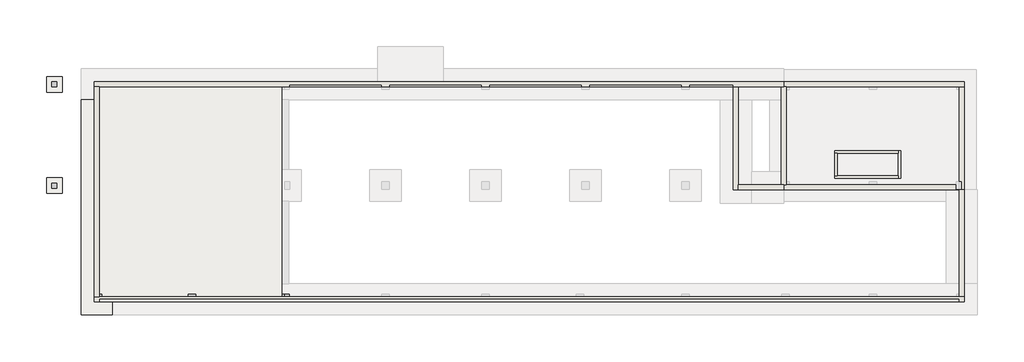
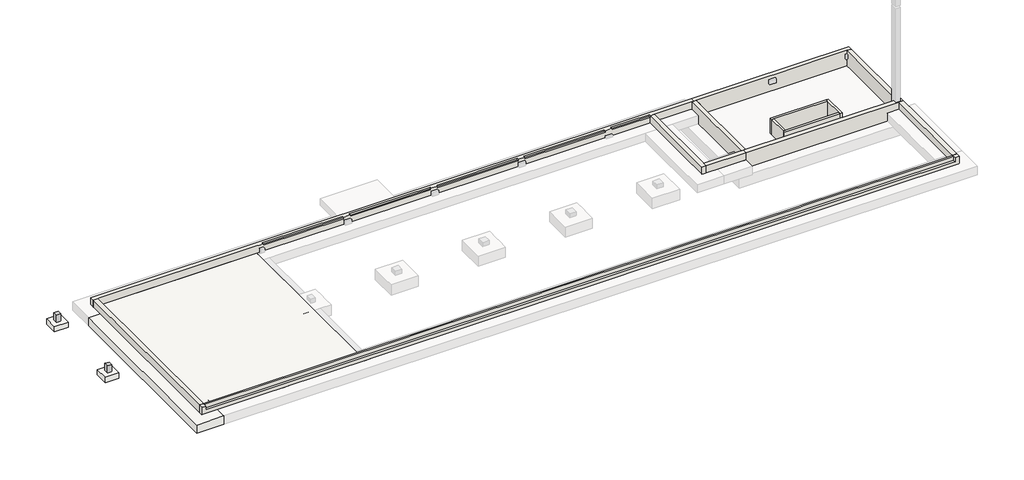
# Not in any storey, part 1 of 2: 14 walls, 5 columns, 3 slabs, 2 beams, 1 footing.
"""IFC4 building model written with IfcOpenShell, lengths in millimetres."""

import ifcopenshell
import ifcopenshell.guid

model = None  # the IFC model being written
_history = None  # IfcOwnerHistory: only IFC2X3 demands one
_inside = {}  # id of a spatial element -> (the spatial element, [elements in it])
_under = {}  # id of a project, library or spatial element -> (it, [spatial elements below it])
_declared = {}  # id of a project -> (the project, [libraries it declares])
_typed = {}  # id of a type object -> (the type object, [elements of that type])
_made_of = {}  # id of a material, layer set ... -> (it, [elements and type objects made of it])


def new_model(schema):
    """Start an empty IFC model of exactly this schema.

    Asked for "IFC4X3", IfcOpenShell would pick the latest addendum, in which some entities
    have other attributes; the version numbers below select the first issue.
    IFC2X3 requires an IfcOwnerHistory on every rooted entity: one is made here for all.
    """
    global model, _history
    if schema == "IFC4X3":
        model = ifcopenshell.file(schema_version=(4, 3, 0, 0))
    else:
        model = ifcopenshell.file(schema=schema)
    _inside.clear()
    _under.clear()
    _declared.clear()
    _typed.clear()
    _made_of.clear()
    _history = None
    if model.schema == "IFC2X3":
        org = make("IfcOrganization", Name="unknown")
        user = make(
            "IfcPersonAndOrganization",
            ThePerson=make("IfcPerson", FamilyName="unknown"),
            TheOrganization=org,
        )
        app = make(
            "IfcApplication",
            ApplicationDeveloper=org,
            Version="unknown",
            ApplicationFullName="unknown",
            ApplicationIdentifier="unknown",
        )
        _history = make(
            "IfcOwnerHistory",
            OwningUser=user,
            OwningApplication=app,
            ChangeAction="ADDED",
            CreationDate=0,
        )
    return model


def make(cls, **values):
    """One entity of the class cls with the attributes given. An attribute that is None is left unset."""
    return model.create_entity(
        cls, **{name: value for name, value in values.items() if value is not None}
    )


def rooted(cls, **values):
    """An entity with a GlobalId (a new one), such as an element, a storey or a relation."""
    return make(cls, GlobalId=ifcopenshell.guid.new(), OwnerHistory=_history, **values)


def si_unit(unit_type, name, prefix=None):
    """IfcSIUnit, for example si_unit("LENGTHUNIT", "METRE", prefix="MILLI")."""
    return make("IfcSIUnit", UnitType=unit_type, Prefix=prefix, Name=name)


def assignment(units):
    """IfcUnitAssignment: the units of a project."""
    return None if units is None else make("IfcUnitAssignment", Units=units)


def point(xyz):
    """IfcCartesianPoint."""
    return None if xyz is None else make("IfcCartesianPoint", Coordinates=xyz)


def direction(xyz):
    """IfcDirection."""
    return None if xyz is None else make("IfcDirection", DirectionRatios=xyz)


def frame(location, z_axis=None, x_axis=None):
    """IfcAxis2Placement3D, a coordinate frame: its origin and axes. An axis left out is left unset."""
    return make(
        "IfcAxis2Placement3D",
        Location=point(location),
        Axis=direction(z_axis),
        RefDirection=direction(x_axis),
    )


def origin():
    """The frame at (0, 0, 0) with its axes left unset."""
    return frame((0.0, 0.0, 0.0))


def place(relative_to, where):
    """IfcLocalPlacement: puts the frame where relative to a parent placement (None: the world)."""
    return make(
        "IfcLocalPlacement", PlacementRelTo=relative_to, RelativePlacement=where
    )


def context(
    kind, dimensions, precision=None, world=None, true_north=None, identifier=None
):
    """IfcGeometricRepresentationContext, for example the 3D "Model" context."""
    return make(
        "IfcGeometricRepresentationContext",
        ContextIdentifier=identifier,
        ContextType=kind,
        CoordinateSpaceDimension=dimensions,
        Precision=precision,
        WorldCoordinateSystem=world,
        TrueNorth=true_north,
    )


def project(units=None, contexts=None):
    """IfcProject with its units and contexts."""
    return rooted(
        "IfcProject",
        Name="project",
        RepresentationContexts=contexts,
        UnitsInContext=assignment(units),
    )


def spatial(cls, under=None, at=None, **own):
    """A site, building, storey or space (cls), placed at a placement, below another one or the project."""
    s = rooted(cls, ObjectPlacement=at, **own)
    if under is not None:
        _under.setdefault(under.id(), (under, []))[1].append(s)
    return s


def polyline(points):
    """IfcPolyline through the points."""
    return make("IfcPolyline", Points=[point(p) for p in points])


def outline(outer, holes=None, kind="AREA"):
    """IfcArbitraryClosedProfileDef: a profile drawn as a closed curve; with holes, ...WithVoids."""
    if holes is None:
        return make("IfcArbitraryClosedProfileDef", ProfileType=kind, OuterCurve=outer)
    return make(
        "IfcArbitraryProfileDefWithVoids",
        ProfileType=kind,
        OuterCurve=outer,
        InnerCurves=holes,
    )


def extrude(swept, where, along, depth):
    """IfcExtrudedAreaSolid: the profile swept, set in the frame where, extruded along a direction by depth."""
    return make(
        "IfcExtrudedAreaSolid",
        SweptArea=swept,
        Position=where,
        ExtrudedDirection=direction(along),
        Depth=depth,
    )


def faces_of(points, faces, orient=None, outer=None):
    """IfcFace entities. A face is a list of loops; a loop is a list of indices into points, from 0.

    orient and outer hold one flag for each loop. By default every Orientation is true, the
    first loop of a face is its IfcFaceOuterBound and the others are IfcFaceBound.
    """
    made = []
    for i, loops in enumerate(faces):
        bounds = []
        for j, loop in enumerate(loops):
            is_outer = j == 0 if outer is None else outer[i][j]
            bounds.append(
                make(
                    "IfcFaceOuterBound" if is_outer else "IfcFaceBound",
                    Bound=make("IfcPolyLoop", Polygon=[points[k] for k in loop]),
                    Orientation=True if orient is None else orient[i][j],
                )
            )
        made.append(make("IfcFace", Bounds=bounds))
    return made


def faceted_brep(points, faces, orient=None, outer=None, voids=None):
    """IfcFacetedBrep: a solid bounded by flat faces; with voids (closed shells), ...WithVoids."""
    shared = [point(p) for p in points]
    hull = make("IfcClosedShell", CfsFaces=faces_of(shared, faces, orient, outer))
    if voids is None:
        return make("IfcFacetedBrep", Outer=hull)
    return make(
        "IfcFacetedBrepWithVoids",
        Outer=hull,
        Voids=[
            make(cls, CfsFaces=faces_of(shared, fs, o, b)) for cls, fs, o, b in voids
        ],
    )


def shape(context_of_items, identifier, shape_type, items):
    """IfcShapeRepresentation: the items that make up one representation, for example the "Body"."""
    return make(
        "IfcShapeRepresentation",
        ContextOfItems=context_of_items,
        RepresentationIdentifier=identifier,
        RepresentationType=shape_type,
        Items=items,
    )


def source(mapping_origin, context_of_items, identifier, shape_type, items):
    """IfcRepresentationMap: a shape defined once, which mapped items show again and again."""
    return make(
        "IfcRepresentationMap",
        MappingOrigin=mapping_origin,
        MappedRepresentation=shape(context_of_items, identifier, shape_type, items),
    )


def transform(
    local_origin,
    x_axis=None,
    y_axis=None,
    z_axis=None,
    scale=None,
    scale2=None,
    scale3=None,
    uniform=True,
):
    """IfcCartesianTransformationOperator3D, or its non-uniform kind. x_axis, y_axis, z_axis: its Axis1, 2, 3."""
    if uniform:
        return make(
            "IfcCartesianTransformationOperator3D",
            Axis1=direction(x_axis),
            Axis2=direction(y_axis),
            LocalOrigin=point(local_origin),
            Scale=scale,
            Axis3=direction(z_axis),
        )
    return make(
        "IfcCartesianTransformationOperator3DnonUniform",
        Axis1=direction(x_axis),
        Axis2=direction(y_axis),
        LocalOrigin=point(local_origin),
        Scale=scale,
        Axis3=direction(z_axis),
        Scale2=scale2,
        Scale3=scale3,
    )


def mapped(mapping_source, mapping_target):
    """IfcMappedItem: shows the shape of a source again, moved by a transform."""
    return make(
        "IfcMappedItem", MappingSource=mapping_source, MappingTarget=mapping_target
    )


def made_of(thing, what):
    """Note that an element or type object is made of a material, layer set ...; save() writes the relation."""
    if what is not None:
        _made_of.setdefault(what.id(), (what, []))[1].append(thing)
    return thing


def element(
    cls,
    number,
    at=None,
    inside=None,
    cuts=None,
    type_object=None,
    material=None,
    context=None,
    identifier="Body",
    shape_type=None,
    held_by="IfcProductDefinitionShape",
    body=None,
    shapes=None,
    **own,
):
    """One element of the class cls, such as IfcWall. Its Tag is "e" and its number.

    at: its placement. inside: the storey or other place that contains it. cuts: it is an
    opening in that element (IfcRelVoidsElement). A single representation is given by context,
    identifier, shape_type and body (its items); several are given by shapes. held_by: the class
    of the entity that holds the representations. save() writes the other relations.
    """
    e = rooted(cls, Tag="e%d" % number, ObjectPlacement=at, **own)
    if body is not None:
        shapes = [shape(context, identifier, shape_type, body)]
    if shapes is not None:
        e.Representation = make(held_by, Representations=shapes)
    if inside is not None:
        _inside.setdefault(inside.id(), (inside, []))[1].append(e)
    if cuts is not None:
        rooted(
            "IfcRelVoidsElement", RelatingBuildingElement=cuts, RelatedOpeningElement=e
        )
    if type_object is not None:
        _typed.setdefault(type_object.id(), (type_object, []))[1].append(e)
    return made_of(e, material)


def aggregate(whole, parts):
    """IfcRelAggregates: a whole, such as a stair, and the parts it consists of."""
    return rooted("IfcRelAggregates", RelatingObject=whole, RelatedObjects=parts)


def save(model, path):
    """Write the relations noted so far, then the file.

    IfcRelAggregates (storeys below a building ...), IfcRelContainedInSpatialStructure (elements
    in a storey), IfcRelDefinesByType, IfcRelAssociatesMaterial and IfcRelDeclares: one each for
    every whole, place, type object, material and project.
    """
    for whole, parts in _under.values():
        aggregate(whole, parts)
    for where, things in _inside.values():
        rooted(
            "IfcRelContainedInSpatialStructure",
            RelatedElements=things,
            RelatingStructure=where,
        )
    for kind, things in _typed.values():
        rooted("IfcRelDefinesByType", RelatedObjects=things, RelatingType=kind)
    for what, things in _made_of.values():
        rooted("IfcRelAssociatesMaterial", RelatedObjects=things, RelatingMaterial=what)
    for by, libraries in _declared.values():
        rooted("IfcRelDeclares", RelatingContext=by, RelatedDefinitions=libraries)
    model.write(path)


def foundation_rectangular_non_pile_17b72d6a(model_context):
    return source(origin(), model_context, "Body", "SweptSolid", [
        extrude(outline(polyline([(625.0, 625.0), (625.0, -625.0), (-625.0, -625.0), (-625.0, 625.0), (625.0, 625.0)])), frame((0.0, 0.0, -500.0), z_axis=(0.0, 0.0, 1.0), x_axis=(1.0, 0.0, 0.0)), (0.0, 0.0, 1.0), 500.0),
    ])


model = new_model("IFC4")

# Units and contexts
model_context = context("Model", 3, world=origin())
ifc_project = project(units=[si_unit("LENGTHUNIT", "METRE", prefix="MILLI")], contexts=[model_context])

# Site, building
site = spatial("IfcSite", under=ifc_project)
building = spatial("IfcBuilding", under=site)

# Beams
placement = place(None, origin())
element("IfcBeam", 1, ObjectType="RC Beam_Rectangular : H_SB_AR_S16_TG_B500xH700_FB1", at=placement, inside=building, context=model_context, shape_type="SweptSolid", body=[
    extrude(outline(polyline([(3500.0, 9199.5208589), (4000.0, 9199.5208589), (4000.0, 1649.5208589), (3500.0, 1649.5208589), (3500.0, 9199.5208589)])), frame((0.0, 0.0, -1250.0381366), z_axis=(0.0, 0.0, 1.0), x_axis=(1.0, 0.0, 0.0)), (0.0, 0.0, 1.0), 550.0),
])
element("IfcBeam", 2, ObjectType="RC Beam_Rectangular : H_SB_AR_S16_TG_B500xH700_FG1", at=placement, inside=building, context=model_context, shape_type="SweptSolid", body=[
    extrude(outline(polyline([(7750.0, 1649.5208589), (7250.0, 1649.5208589), (7250.0, 8249.5208589), (7750.0, 8249.5208589), (7750.0, 1649.5208589)])), frame((0.0, 0.0, -1250.0381366), z_axis=(0.0, 0.0, 1.0), x_axis=(1.0, 0.0, 0.0)), (0.0, 0.0, 1.0), 550.0),
])

# Columns
element("IfcColumn", 3, ObjectType="RC_Column_Rectangular : H_SC_AR_S15_UG_W600xL600_C2", at=placement, inside=building, context=model_context, shape_type="Brep", body=[
    faceted_brep([(15300.0, 799.5208589, -850.0381366), (15300.0, 199.5208589, -850.0381366), (14700.0, 199.5208589, -850.0381366), (14700.0, 799.5208589, -850.0381366), (15300.0, 799.5208589, -150.0381366), (15300.0, 599.5208589, -150.0381366), (15300.0, 599.5208589, -550.0381366), (15300.0, 199.5208589, -550.0381366), (14700.0, 199.5208589, -550.0381366), (14700.0, 599.5208589, -550.0381366), (14700.0, 799.5208589, -550.0381366), (14950.0, 799.5208589, -550.0381366), (14950.0, 799.5208589, -150.0381366), (14950.0, 599.5208589, -150.0381366), (14950.0, 599.5208589, -550.0381366)], [[[0, 1, 2, 3]], [[1, 0, 4, 5, 6, 7]], [[2, 1, 7, 8]], [[3, 2, 8, 9, 10]], [[0, 3, 10, 11, 12, 4]], [[5, 4, 12, 13]], [[6, 5, 13, 14]], [[7, 6, 14, 11, 10, 9, 8]], [[11, 14, 13, 12]]]),
])
element("IfcColumn", 4, ObjectType="RC_Column_Rectangular : H_SC_AR_S15_UG_W600xL600_C2", at=placement, inside=building, context=model_context, shape_type="Brep", body=[
    faceted_brep([(7800.0, 799.5208589, -850.0381366), (7800.0, 199.5208589, -850.0381366), (7200.0, 199.5208589, -850.0381366), (7200.0, 799.5208589, -850.0381366), (7800.0, 599.5208589, -150.0381366), (7800.0, 599.5208589, -550.0381366), (7800.0, 799.5208589, -550.0381366), (7800.0, 799.5208589, -150.0381366), (7800.0, 199.5208589, -550.0381366), (7200.0, 199.5208589, -550.0381366), (7200.0, 599.5208589, -550.0381366), (7200.0, 599.5208589, -150.0381366), (7200.0, 799.5208589, -150.0381366), (7200.0, 799.5208589, -550.0381366), (7200.0, 599.5208589, -700.0381366), (7800.0, 599.5208589, -700.0381366), (7800.0, 799.5208589, -700.0381366), (7200.0, 799.5208589, -700.0381366)], [[[0, 1, 2, 3]], [[4, 5, 6, 7]], [[2, 1, 8, 9]], [[10, 11, 12, 13]], [[12, 7, 6, 13]], [[7, 12, 11, 4]], [[10, 5, 4, 11]], [[5, 10, 9, 8]], [[14, 15, 16, 17]], [[5, 10, 13, 6]], [[10, 5, 15, 14]], [[1, 0, 16, 15, 5, 8]], [[3, 2, 9, 10, 14, 17]], [[0, 3, 17, 16]]]),
])
element("IfcColumn", 5, ObjectType="RC_Column_Rectangular : H_SC_AR_S15_UG_W600xL600_C2", at=placement, inside=building, context=model_context, shape_type="Brep", body=[
    faceted_brep([(300.0, 799.5208589, -850.0381366), (300.0, 199.5208589, -850.0381366), (-300.0, 199.5208589, -850.0381366), (-300.0, 799.5208589, -850.0381366), (300.0, 599.5208589, -150.0381366), (300.0, 599.5208589, -550.0381366), (300.0, 799.5208589, -550.0381366), (300.0, 799.5208589, -150.0381366), (300.0, 199.5208589, -550.0381366), (-300.0, 199.5208589, -550.0381366), (-300.0, 599.5208589, -550.0381366), (-300.0, 799.5208589, -550.0381366), (100.0, 799.5208589, -550.0381366), (100.0, 799.5208589, -150.0381366), (100.0, 599.5208589, -150.0381366), (100.0, 599.5208589, -550.0381366), (100.0, 799.5208589, -700.0381366), (100.0, 599.5208589, -700.0381366), (300.0, 599.5208589, -700.0381366), (300.0, 799.5208589, -700.0381366), (100.0, 599.5208589, -550.0381366)], [[[0, 1, 2, 3]], [[4, 5, 6, 7]], [[2, 1, 8, 9]], [[3, 2, 9, 10, 11]], [[12, 13, 7, 6]], [[4, 7, 13, 14]], [[5, 4, 14, 15]], [[8, 5, 15, 12, 11, 10, 9]], [[12, 15, 14, 13]], [[16, 17, 18, 19]], [[5, 20, 12, 6]], [[17, 20, 5, 18]], [[20, 17, 16, 12]], [[1, 0, 19, 18, 5, 8]], [[0, 3, 11, 12, 16, 19]]]),
])
element("IfcColumn", 6, ObjectType="RC_Column_Rectangular : H_SC_AR_S15_UG_W400xL400_C3", at=placement, inside=building, context=model_context, shape_type="SweptSolid", body=[
    extrude(outline(polyline([(-3300.0, 9699.5208589), (-3300.0, 9299.5208589), (-3700.0, 9299.5208589), (-3700.0, 9699.5208589), (-3300.0, 9699.5208589)])), frame((0.0, 0.0, -850.0381366), z_axis=(0.0, 0.0, 1.0), x_axis=(1.0, 0.0, 0.0)), (0.0, 0.0, 1.0), 700.0),
])
element("IfcColumn", 7, ObjectType="RC_Column_Rectangular : H_SC_AR_S15_UG_W400xL400_C3", at=placement, inside=building, context=model_context, shape_type="Brep", body=[
    faceted_brep([(-3300.0, 17799.5208589, -850.0381366), (-3300.0, 17399.5208589, -850.0381366), (-3700.0, 17399.5208589, -850.0381366), (-3700.0, 17799.5208589, -850.0381366), (-3300.0, 17799.5208589, -150.0381366), (-3300.0, 17399.5208589, -150.0381366), (-3300.0, 17399.5208589, -550.0381366), (-3300.0, 17799.5208589, -550.0381366), (-3700.0, 17399.5208589, -150.0381366), (-3700.0, 17799.5208589, -150.0381366)], [[[0, 1, 2, 3]], [[4, 5, 6, 1, 0, 7]], [[5, 8, 2, 1, 6]], [[8, 9, 3, 2]], [[9, 4, 7, 0, 3]], [[4, 9, 8, 5]]]),
])

# Footing
element("IfcFooting", 8, ObjectType="H_SF_AR_S18_Wall FDN_T800", at=placement, inside=building, context=model_context, shape_type="Brep", body=[
    faceted_brep([(-1350.0, -850.4791411, -550.0381366), (1150.0, -850.4791411, -550.0381366), (1150.0, 1649.5208589, -550.0381366), (1150.0, 16349.5208589, -550.0381366), (-1350.0, 16349.5208589, -550.0381366), (-1350.0, -850.4791411, -1350.0381366), (-1350.0, 16349.5208589, -1350.0381366), (1150.0, -850.4791411, -1350.0381366), (1150.0, 16349.5208589, -1350.0381366), (1150.0, 9799.5208589, -1350.0381366), (1150.0, 9199.5208589, -1350.0381366), (1150.0, 1649.5208589, -1350.0381366)], [[[0, 1, 2, 3, 4]], [[5, 0, 4, 6]], [[7, 5, 6, 8, 9, 10, 11]], [[1, 7, 11, 10, 9, 8, 3, 2]], [[1, 0, 5, 7]], [[4, 3, 8, 6]]]),
])

# Slabs
element("IfcSlab", 9, ObjectType="H_FL_AR_S17_RC Slab T150_B1S1", at=placement, inside=building, context=model_context, shape_type="Brep", body=[
    faceted_brep([(14700.0, 17399.5208589, -700.0381366), (14700.0, 599.5208589, -700.0381366), (7800.0, 599.5208589, -700.0381366), (7200.0, 599.5208589, -700.0381366), (300.0, 599.5208589, -700.0381366), (100.0, 599.5208589, -700.0381366), (100.0, 799.5208589, -700.0381366), (100.0, 17199.5208589, -700.0381366), (100.0, 17399.5208589, -700.0381366), (300.0, 17399.5208589, -700.0381366), (7200.0, 17399.5208589, -700.0381366), (7800.0, 17399.5208589, -700.0381366), (14700.0, 17399.5208589, -550.0381366), (7800.0, 17399.5208589, -550.0381366), (7200.0, 17399.5208589, -550.0381366), (300.0, 17399.5208589, -550.0381366), (100.0, 17399.5208589, -550.0381366), (100.0, 17199.5208589, -550.0381366), (100.0, 799.5208589, -550.0381366), (100.0, 599.5208589, -550.0381366), (300.0, 599.5208589, -550.0381366), (7200.0, 599.5208589, -550.0381366), (7800.0, 599.5208589, -550.0381366), (14700.0, 599.5208589, -550.0381366), (14700.0, 799.5208589, -550.0381366), (14700.0, 17199.5208589, -550.0381366)], [[[0, 1, 2, 3, 4, 5, 6, 7, 8, 9, 10, 11]], [[12, 13, 14, 15, 16, 17, 18, 19, 20, 21, 22, 23, 24, 25]], [[1, 0, 12, 25, 24, 23]], [[5, 4, 3, 2, 1, 23, 22, 21, 20, 19]], [[8, 7, 6, 5, 19, 18, 17, 16]], [[0, 11, 10, 9, 8, 16, 15, 14, 13, 12]]]),
])
element("IfcSlab", 10, ObjectType="Foundation Rectangular (Non-Pile) : H_SF_AR_S18_W1250xL1250xT500_Bitumen_F2", at=placement, inside=building, context=model_context, shape_type="SweptSolid", body=[
    extrude(outline(polyline([(-2875.0, 18224.5208589), (-2875.0, 16974.5208589), (-4125.0, 16974.5208589), (-4125.0, 18224.5208589), (-2875.0, 18224.5208589)])), frame((0.0, 0.0, -1350.0381366), z_axis=(0.0, 0.0, 1.0), x_axis=(1.0, 0.0, 0.0)), (0.0, 0.0, 1.0), 500.0),
])
foundation_rectangular_non_pile_shape = foundation_rectangular_non_pile_17b72d6a(model_context)
element("IfcSlab", 11, ObjectType="Foundation Rectangular (Non-Pile) : H_SF_AR_S18_W1250xL1250xT500_Bitumen_F2", at=placement, inside=building, context=model_context, shape_type="MappedRepresentation", body=[
    mapped(foundation_rectangular_non_pile_shape, transform((-3500.0, 9499.5208589, -850.0381366), x_axis=(1.0, 0.0, 0.0), y_axis=(0.0, 1.0, 0.0), z_axis=(0.0, 0.0, 1.0))),
])

# Walls
element("IfcWall", 12, ObjectType="H_WA_AR_B02_Ext Wall_RC T400_UG_Bitumen 2", at=placement, inside=building, context=model_context, shape_type="Brep", body=[
    faceted_brep([(-300.0, 17399.5208589, -550.0381366), (100.0, 17399.5208589, -550.0381366), (300.0, 17399.5208589, -550.0381366), (7200.0, 17399.5208589, -550.0381366), (7800.0, 17399.5208589, -550.0381366), (14700.0, 17399.5208589, -550.0381366), (14950.0, 17399.5208589, -550.0381366), (15300.0, 17399.5208589, -550.0381366), (22700.0, 17399.5208589, -550.0381366), (23300.0, 17399.5208589, -550.0381366), (30700.0, 17399.5208589, -550.0381366), (31300.0, 17399.5208589, -550.0381366), (38700.0, 17399.5208589, -550.0381366), (39300.0, 17399.5208589, -550.0381366), (46700.0, 17399.5208589, -550.0381366), (47300.0, 17399.5208589, -550.0381366), (50825.0, 17399.5208589, -550.0381366), (51225.0, 17399.5208589, -550.0381366), (54650.0, 17399.5208589, -550.0381366), (54850.0, 17399.5208589, -550.0381366), (54850.0, 17399.5208589, 149.9618634), (54650.0, 17399.5208589, 149.9618634), (51225.0, 17399.5208589, 149.9618634), (50825.0, 17399.5208589, 149.9618634), (50825.0, 17399.5208589, -0.0381366), (47300.0, 17399.5208589, -0.0381366), (47300.0, 17399.5208589, 149.9618634), (46700.0, 17399.5208589, 149.9618634), (46700.0, 17399.5208589, -0.0381366), (39300.0, 17399.5208589, -0.0381366), (39300.0, 17399.5208589, 149.9618634), (38700.0, 17399.5208589, 149.9618634), (38700.0, 17399.5208589, -0.0381366), (31300.0, 17399.5208589, -0.0381366), (31300.0, 17399.5208589, 149.9618634), (30700.0, 17399.5208589, 149.9618634), (30700.0, 17399.5208589, -0.0381366), (23300.0, 17399.5208589, -0.0381366), (23300.0, 17399.5208589, 149.9618634), (22700.0, 17399.5208589, 149.9618634), (22700.0, 17399.5208589, -0.0381366), (15300.0, 17399.5208589, -0.0381366), (15300.0, 17399.5208589, 149.9618634), (14950.0, 17399.5208589, 149.9618634), (14700.0, 17399.5208589, 149.9618634), (7800.0, 17399.5208589, 149.9618634), (7200.0, 17399.5208589, 149.9618634), (300.0, 17399.5208589, 149.9618634), (100.0, 17399.5208589, 149.9618634), (-300.0, 17399.5208589, 149.9618634), (-300.0, 17399.5208589, -20.0381366), (54850.0, 17799.5208589, -550.0381366), (54650.0, 17799.5208589, -550.0381366), (47300.0, 17799.5208589, -550.0381366), (46700.0, 17799.5208589, -550.0381366), (39300.0, 17799.5208589, -550.0381366), (38700.0, 17799.5208589, -550.0381366), (31300.0, 17799.5208589, -550.0381366), (30700.0, 17799.5208589, -550.0381366), (23300.0, 17799.5208589, -550.0381366), (22700.0, 17799.5208589, -550.0381366), (15300.0, 17799.5208589, -550.0381366), (14700.0, 17799.5208589, -550.0381366), (7800.0, 17799.5208589, -550.0381366), (7200.0, 17799.5208589, -550.0381366), (300.0, 17799.5208589, -550.0381366), (-300.0, 17799.5208589, -550.0381366), (-300.0, 17799.5208589, -20.0381366), (-300.0, 17799.5208589, 149.9618634), (18450.0, 17799.5208589, 149.9618634), (19550.0, 17799.5208589, 149.9618634), (24050.0, 17799.5208589, 149.9618634), (26150.0, 17799.5208589, 149.9618634), (54850.0, 17799.5208589, 149.9618634), (-300.0, 17549.5208589, 149.9618634), (15300.0, 17549.5208589, 149.9618634), (22700.0, 17549.5208589, 149.9618634), (23300.0, 17549.5208589, 149.9618634), (30700.0, 17549.5208589, 149.9618634), (31300.0, 17549.5208589, 149.9618634), (38700.0, 17549.5208589, 149.9618634), (39300.0, 17549.5208589, 149.9618634), (46700.0, 17549.5208589, 149.9618634), (47300.0, 17549.5208589, 149.9618634), (50825.0, 17549.5208589, 149.9618634), (22700.0, 17549.5208589, -0.0381366), (15300.0, 17549.5208589, -0.0381366), (30700.0, 17549.5208589, -0.0381366), (23300.0, 17549.5208589, -0.0381366), (38700.0, 17549.5208589, -0.0381366), (31300.0, 17549.5208589, -0.0381366), (46700.0, 17549.5208589, -0.0381366), (39300.0, 17549.5208589, -0.0381366), (50825.0, 17549.5208589, -0.0381366), (47300.0, 17549.5208589, -0.0381366)], [[[0, 1, 2, 3, 4, 5, 6, 7, 8, 9, 10, 11, 12, 13, 14, 15, 16, 17, 18, 19, 20, 21, 22, 23, 24, 25, 26, 27, 28, 29, 30, 31, 32, 33, 34, 35, 36, 37, 38, 39, 40, 41, 42, 43, 44, 45, 46, 47, 48, 49, 50]], [[51, 52, 53, 54, 55, 56, 57, 58, 59, 60, 61, 62, 63, 64, 65, 66, 67, 68, 69, 70, 71, 72, 73]], [[19, 18, 17, 16, 15, 14, 13, 12, 11, 10, 9, 8, 7, 6, 5, 4, 3, 2, 1, 0, 66, 65, 64, 63, 62, 61, 60, 59, 58, 57, 56, 55, 54, 53, 52, 51]], [[20, 19, 51, 73]], [[73, 72, 71, 70, 69, 68, 74, 49, 48, 47, 46, 45, 44, 43, 42, 75, 76, 39, 38, 77, 78, 35, 34, 79, 80, 31, 30, 81, 82, 27, 26, 83, 84, 23, 22, 21, 20]], [[49, 74, 68, 67, 66, 0, 50]], [[85, 86, 41, 40]], [[87, 88, 37, 36]], [[89, 90, 33, 32]], [[91, 92, 29, 28]], [[93, 94, 25, 24]], [[86, 75, 42, 41]], [[86, 85, 76, 75]], [[76, 85, 40, 39]], [[88, 77, 38, 37]], [[88, 87, 78, 77]], [[78, 87, 36, 35]], [[90, 79, 34, 33]], [[90, 89, 80, 79]], [[80, 89, 32, 31]], [[92, 81, 30, 29]], [[92, 91, 82, 81]], [[82, 91, 28, 27]], [[94, 83, 26, 25]], [[94, 93, 84, 83]], [[84, 93, 24, 23]]]),
])
element("IfcWall", 13, ObjectType="H_WA_AR_B02_Ext Wall_RC T400_UG_Bitumen 2", at=placement, inside=building, context=model_context, shape_type="Brep", body=[
    faceted_brep([(69300.0, 599.5208589, -550.0381366), (68900.0, 599.5208589, -550.0381366), (68700.0, 599.5208589, -550.0381366), (62300.0, 599.5208589, -550.0381366), (61700.0, 599.5208589, -550.0381366), (55300.0, 599.5208589, -550.0381366), (54700.0, 599.5208589, -550.0381366), (47300.0, 599.5208589, -550.0381366), (46700.0, 599.5208589, -550.0381366), (39240.1112654, 599.5208589, -550.0381366), (38850.0, 599.5208589, -550.0381366), (38250.0, 599.5208589, -550.0381366), (31300.0, 599.5208589, -550.0381366), (30700.0, 599.5208589, -550.0381366), (23300.0, 599.5208589, -550.0381366), (22700.0, 599.5208589, -550.0381366), (15300.0, 599.5208589, -550.0381366), (14950.0, 599.5208589, -550.0381366), (14700.0, 599.5208589, -550.0381366), (7800.0, 599.5208589, -550.0381366), (7200.0, 599.5208589, -550.0381366), (300.0, 599.5208589, -550.0381366), (100.0, 599.5208589, -550.0381366), (-300.0, 599.5208589, -550.0381366), (-300.0, 599.5208589, 149.9618634), (100.0, 599.5208589, 149.9618634), (300.0, 599.5208589, 149.9618634), (7200.0, 599.5208589, 149.9618634), (7800.0, 599.5208589, 149.9618634), (14700.0, 599.5208589, 149.9618634), (14950.0, 599.5208589, 149.9618634), (15300.0, 599.5208589, 149.9618634), (22700.0, 599.5208589, 149.9618634), (23300.0, 599.5208589, 149.9618634), (30700.0, 599.5208589, 149.9618634), (31300.0, 599.5208589, 149.9618634), (38700.0, 599.5208589, 149.9618634), (39300.0, 599.5208589, 149.9618634), (46700.0, 599.5208589, 149.9618634), (47300.0, 599.5208589, 149.9618634), (54700.0, 599.5208589, 149.9618634), (55300.0, 599.5208589, 149.9618634), (61700.0, 599.5208589, 149.9618634), (62300.0, 599.5208589, 149.9618634), (68700.0, 599.5208589, 149.9618634), (68900.0, 599.5208589, 149.9618634), (69300.0, 599.5208589, 149.9618634), (-300.0, 199.5208589, -550.0381366), (300.0, 199.5208589, -550.0381366), (7200.0, 199.5208589, -550.0381366), (7800.0, 199.5208589, -550.0381366), (14700.0, 199.5208589, -550.0381366), (15300.0, 199.5208589, -550.0381366), (22700.0, 199.5208589, -550.0381366), (23300.0, 199.5208589, -550.0381366), (30700.0, 199.5208589, -550.0381366), (31300.0, 199.5208589, -550.0381366), (38250.0, 199.5208589, -550.0381366), (38850.0, 199.5208589, -550.0381366), (46700.0, 199.5208589, -550.0381366), (47300.0, 199.5208589, -550.0381366), (54700.0, 199.5208589, -550.0381366), (55300.0, 199.5208589, -550.0381366), (61700.0, 199.5208589, -550.0381366), (62300.0, 199.5208589, -550.0381366), (68700.0, 199.5208589, -550.0381366), (69300.0, 199.5208589, -550.0381366), (69300.0, 199.5208589, 149.9618634), (68900.0, 199.5208589, 149.9618634), (68900.0, 199.5208589, -231.142699), (100.0, 199.5208589, -231.142699), (100.0, 199.5208589, 149.9618634), (-50.0, 199.5208589, 149.9618634), (-300.0, 199.5208589, 149.9618634), (100.0, 449.5208589, 149.9618634), (300.0, 449.5208589, 149.9618634), (7200.0, 449.5208589, 149.9618634), (7800.0, 449.5208589, 149.9618634), (14700.0, 449.5208589, 149.9618634), (15300.0, 449.5208589, 149.9618634), (22700.0, 449.5208589, 149.9618634), (23300.0, 449.5208589, 149.9618634), (30700.0, 449.5208589, 149.9618634), (31300.0, 449.5208589, 149.9618634), (38700.0, 449.5208589, 149.9618634), (39300.0, 449.5208589, 149.9618634), (46700.0, 449.5208589, 149.9618634), (47300.0, 449.5208589, 149.9618634), (53150.0, 449.5208589, 149.9618634), (54150.0, 449.5208589, 149.9618634), (54700.0, 449.5208589, 149.9618634), (55300.0, 449.5208589, 149.9618634), (61700.0, 449.5208589, 149.9618634), (62300.0, 449.5208589, 149.9618634), (68700.0, 449.5208589, 149.9618634), (68900.0, 449.5208589, 149.9618634), (69300.0, 449.5208589, 149.9618634), (100.0, 449.5208589, -231.142699), (68900.0, 449.5208589, -231.142699)], [[[0, 1, 2, 3, 4, 5, 6, 7, 8, 9, 10, 11, 12, 13, 14, 15, 16, 17, 18, 19, 20, 21, 22, 23, 24, 25, 26, 27, 28, 29, 30, 31, 32, 33, 34, 35, 36, 37, 38, 39, 40, 41, 42, 43, 44, 45, 46]], [[47, 48, 49, 50, 51, 52, 53, 54, 55, 56, 57, 58, 59, 60, 61, 62, 63, 64, 65, 66, 67, 68, 69, 70, 71, 72, 73]], [[23, 22, 21, 20, 19, 18, 17, 16, 15, 14, 13, 12, 11, 10, 9, 8, 7, 6, 5, 4, 3, 2, 1, 0, 66, 65, 64, 63, 62, 61, 60, 59, 58, 57, 56, 55, 54, 53, 52, 51, 50, 49, 48, 47]], [[46, 45, 44, 43, 42, 41, 40, 39, 38, 37, 36, 35, 34, 33, 32, 31, 30, 29, 28, 27, 26, 25, 24, 73, 72, 71, 74, 75, 76, 77, 78, 79, 80, 81, 82, 83, 84, 85, 86, 87, 88, 89, 90, 91, 92, 93, 94, 95, 68, 67, 96]], [[23, 47, 73, 24]], [[66, 0, 46, 96, 67]], [[97, 98, 95, 94, 93, 92, 91, 90, 89, 88, 87, 86, 85, 84, 83, 82, 81, 80, 79, 78, 77, 76, 75, 74]], [[98, 97, 70, 69]], [[97, 74, 71, 70]], [[95, 98, 69, 68]]]),
])
element("IfcWall", 14, ObjectType="H_WA_AR_B02_Ext Wall_RC T400_UG_Bitumen 2", at=placement, inside=building, context=model_context, shape_type="Brep", body=[
    faceted_brep([(100.0, 599.5208589, 149.9618634), (100.0, 599.5208589, -150.0381366), (100.0, 599.5208589, -550.0381366), (100.0, 799.5208589, -550.0381366), (100.0, 17199.5208589, -550.0381366), (100.0, 17399.5208589, -550.0381366), (100.0, 17399.5208589, -150.0381366), (100.0, 17399.5208589, 149.9618634), (100.0, 17199.5208589, 149.9618634), (100.0, 9849.5208589, 149.9618634), (100.0, 9149.5208589, 149.9618634), (100.0, 799.5208589, 149.9618634), (-300.0, 599.5208589, -550.0381366), (-300.0, 599.5208589, 149.9618634), (-300.0, 17399.5208589, 149.9618634), (-300.0, 17399.5208589, -550.0381366), (-300.0, 17199.5208589, -550.0381366), (-300.0, 9699.5208589, -550.0381366), (-300.0, 9299.5208589, -550.0381366), (-300.0, 799.5208589, -550.0381366)], [[[0, 1, 2, 3, 4, 5, 6, 7, 8, 9, 10, 11]], [[12, 13, 14, 15, 16, 17, 18, 19]], [[5, 4, 3, 2, 12, 19, 18, 17, 16, 15]], [[0, 11, 10, 9, 8, 7, 14, 13]], [[5, 15, 14, 7, 6]], [[0, 13, 12, 2, 1]]]),
])
element("IfcWall", 15, ObjectType="H_WA_AR_B02_Ext Wall_RC T400_UG_Bitumen 2", at=placement, inside=building, context=model_context, shape_type="Brep", body=[
    faceted_brep([(68900.0, 9149.5208589, -550.0381366), (68900.0, 799.5208589, -550.0381366), (68900.0, 599.5208589, -550.0381366), (68900.0, 599.5208589, -150.0381366), (68900.0, 599.5208589, 149.9618634), (68900.0, 799.5208589, 149.9618634), (68900.0, 9149.5208589, 149.9618634), (69300.0, 9149.5208589, -550.0381366), (69300.0, 9149.5208589, 149.9618634), (69300.0, 7249.5208589, 149.9618634), (69300.0, 4149.5208589, 149.9618634), (69300.0, 599.5208589, 149.9618634), (69300.0, 599.5208589, -550.0381366), (69300.0, 799.5208589, -550.0381366)], [[[0, 1, 2, 3, 4, 5, 6]], [[7, 8, 9, 10, 11, 12, 13]], [[2, 1, 0, 7, 13, 12]], [[6, 5, 4, 11, 10, 9, 8]], [[0, 6, 8, 7]], [[2, 12, 11, 4, 3]]]),
])
element("IfcWall", 16, ObjectType="H_WA_AR_B02_Ext Wall_RC T400_UG_Bitumen 2", at=placement, inside=building, context=model_context, shape_type="Brep", body=[
    faceted_brep([(50825.0, 17399.5208589, -550.0381366), (50825.0, 9799.5208589, -550.0381366), (50825.0, 9149.5208589, -550.0381366), (50825.0, 9149.5208589, -0.0381366), (50825.0, 9149.5208589, 149.9618634), (50825.0, 9399.5208589, 149.9618634), (50825.0, 17399.5208589, 149.9618634), (51225.0, 17399.5208589, -550.0381366), (51225.0, 17399.5208589, 149.9618634), (51225.0, 9549.5208589, 149.9618634), (51225.0, 9399.5208589, 149.9618634), (51225.0, 9149.5208589, 149.9618634), (51225.0, 9149.5208589, -150.0381366), (51225.0, 9149.5208589, -550.0381366), (51225.0, 9549.5208589, -550.0381366), (51225.0, 9799.5208589, -550.0381366), (51175.0, 9149.5208589, -550.0381366)], [[[0, 1, 2, 3, 4, 5, 6]], [[7, 8, 9, 10, 11, 12, 13, 14, 15]], [[2, 1, 0, 7, 15, 14, 13, 16]], [[6, 5, 4, 11, 10, 9, 8]], [[0, 6, 8, 7]], [[2, 16, 13, 12, 11, 4, 3]]]),
])
element("IfcWall", 17, ObjectType="H_WA_AR_B02_Ext Wall_RC T400_UG_Bitumen 2", at=placement, inside=building, context=model_context, shape_type="Brep", body=[
    faceted_brep([(51225.0, 9149.5208589, 149.9618634), (51225.0, 9149.5208589, -550.0381366), (54650.0, 9149.5208589, -550.0381366), (54700.0, 9149.5208589, -550.0381366), (54850.0, 9149.5208589, -550.0381366), (54850.0, 9149.5208589, 149.9618634), (51225.0, 9549.5208589, -550.0381366), (51225.0, 9549.5208589, -50.0381366), (51225.0, 9549.5208589, 149.9618634), (54650.0, 9549.5208589, 149.9618634), (54850.0, 9549.5208589, 149.9618634), (54850.0, 9549.5208589, -550.0381366), (54650.0, 9549.5208589, -550.0381366)], [[[0, 1, 2, 3, 4, 5]], [[6, 7, 8, 9, 10, 11, 12]], [[4, 3, 2, 1, 6, 12, 11]], [[5, 4, 11, 10]], [[0, 5, 10, 9, 8]], [[0, 8, 7, 6, 1]]]),
])
element("IfcWall", 18, ObjectType="H_WA_AR_B02_Ext Wall_RC T400_UG_Bitumen_W1A", at=placement, inside=building, context=model_context, shape_type="Brep", body=[
    faceted_brep([(54650.0, 17399.5208589, -1350.0381366), (55050.0, 17399.5208589, -1350.0381366), (68900.0, 17399.5208589, -1350.0381366), (69300.0, 17399.5208589, -1350.0381366), (69300.0, 17399.5208589, 149.9618634), (68900.0, 17399.5208589, 149.9618634), (62300.0, 17399.5208589, 149.9618634), (61700.0, 17399.5208589, 149.9618634), (55350.0, 17399.5208589, 149.9618634), (55050.0, 17399.5208589, 149.9618634), (54850.0, 17399.5208589, 149.9618634), (54850.0, 17399.5208589, -150.0381366), (54850.0, 17399.5208589, -550.0381366), (54700.0, 17399.5208589, -550.0381366), (54650.0, 17399.5208589, -550.0381366), (54650.0, 17799.5208589, -1350.0381366), (54650.0, 17799.5208589, -550.0381366), (54850.0, 17799.5208589, -550.0381366), (54850.0, 17799.5208589, 149.9618634), (69300.0, 17799.5208589, 149.9618634), (69300.0, 17799.5208589, -1350.0381366), (54850.0, 17749.5208589, -550.0381366), (54650.0, 17449.5208589, -550.0381366)], [[[0, 1, 2, 3, 4, 5, 6, 7, 8, 9, 10, 11, 12, 13, 14]], [[15, 16, 17, 18, 19, 20]], [[3, 2, 1, 0, 15, 20]], [[10, 9, 8, 7, 6, 5, 4, 19, 18]], [[4, 3, 20, 19]], [[12, 11, 10, 18, 17, 21]], [[12, 21, 17, 16, 22, 14, 13]], [[0, 14, 22, 16, 15]]]),
])
element("IfcWall", 19, ObjectType="H_WA_AR_B02_Ext Wall_RC T400_UG_Bitumen_W1A", at=placement, inside=building, context=model_context, shape_type="Brep", body=[
    faceted_brep([(68900.0, 17399.5208589, -1350.0381366), (68900.0, 9549.5208589, -1350.0381366), (68900.0, 9149.5208589, -1350.0381366), (68900.0, 9149.5208589, -550.0381366), (68900.0, 9149.5208589, 149.9618634), (68900.0, 9549.5208589, 149.9618634), (68900.0, 9799.5208589, 149.9618634), (68900.0, 9849.5208589, 149.9618634), (68900.0, 17399.5208589, 149.9618634), (68900.0, 17399.5208589, -0.0381366), (68900.0, 17399.5208589, -150.0381366), (68900.0, 17399.5208589, -550.0381366), (69300.0, 17399.5208589, -1350.0381366), (69300.0, 17399.5208589, 149.9618634), (69300.0, 9149.5208589, 149.9618634), (69300.0, 9149.5208589, -550.0381366), (69300.0, 9149.5208589, -1350.0381366), (69050.0, 9149.5208589, 149.9618634)], [[[0, 1, 2, 3, 4, 5, 6, 7, 8, 9, 10, 11]], [[12, 13, 14, 15, 16]], [[2, 1, 0, 12, 16]], [[8, 7, 6, 5, 4, 17, 14, 13]], [[0, 11, 10, 9, 8, 13, 12]], [[2, 16, 15, 14, 17, 4, 3]]]),
])
element("IfcWall", 20, ObjectType="H_WA_AR_B02_Ext Wall_RC T400_UG_Bitumen_W1A", at=placement, inside=building, context=model_context, shape_type="Brep", body=[
    faceted_brep([(68900.0, 9549.5208589, 149.9618634), (68900.0, 9549.5208589, -150.0381366), (68900.0, 9549.5208589, -550.0381366), (68900.0, 9549.5208589, -1350.0381366), (55050.0, 9549.5208589, -1350.0381366), (54650.0, 9549.5208589, -1350.0381366), (54650.0, 9549.5208589, -550.0381366), (54850.0, 9549.5208589, -550.0381366), (54850.0, 9549.5208589, 149.9618634), (55050.0, 9549.5208589, 149.9618634), (55350.0, 9549.5208589, 149.9618634), (61650.0, 9549.5208589, 149.9618634), (62350.0, 9549.5208589, 149.9618634), (68600.0, 9549.5208589, 149.9618634), (68650.0, 9549.5208589, 149.9618634), (68900.0, 9149.5208589, -1350.0381366), (68900.0, 9149.5208589, 149.9618634), (68600.0, 9149.5208589, 149.9618634), (54850.0, 9149.5208589, 149.9618634), (54850.0, 9149.5208589, -550.0381366), (54650.0, 9149.5208589, -550.0381366), (54650.0, 9149.5208589, -1350.0381366)], [[[0, 1, 2, 3, 4, 5, 6, 7, 8, 9, 10, 11, 12, 13, 14]], [[15, 16, 17, 18, 19, 20, 21]], [[5, 4, 3, 15, 21]], [[0, 14, 13, 12, 11, 10, 9, 8, 18, 17, 16]], [[8, 7, 19, 18]], [[19, 7, 6, 20]], [[6, 5, 21, 20]], [[0, 16, 15, 3, 2, 1]]]),
])
element("IfcWall", 21, ObjectType="H_WA_AR_B02_Ext Wall_RC T400_UG_Bitumen_W1A", at=placement, inside=building, context=model_context, shape_type="Brep", body=[
    faceted_brep([(55050.0, 9549.5208589, 149.9618634), (55050.0, 9549.5208589, -150.0381366), (55050.0, 9549.5208589, -550.0381366), (55050.0, 9549.5208589, -1350.0381366), (55050.0, 17399.5208589, -1350.0381366), (55050.0, 17399.5208589, -550.0381366), (55050.0, 17399.5208589, -150.0381366), (55050.0, 17399.5208589, 149.9618634), (55050.0, 17099.5208589, 149.9618634), (55050.0, 9849.5208589, 149.9618634), (54650.0, 9549.5208589, -1350.0381366), (54650.0, 9549.5208589, -550.0381366), (54650.0, 9549.5208589, -50.0381366), (54650.0, 9549.5208589, 149.9618634), (54650.0, 17114.5208589, 149.9618634), (54650.0, 17399.5208589, 149.9618634), (54650.0, 17399.5208589, -150.0381366), (54650.0, 17399.5208589, -550.0381366), (54650.0, 17399.5208589, -1350.0381366), (54850.0, 17399.5208589, 149.9618634), (54850.0, 9549.5208589, 149.9618634)], [[[0, 1, 2, 3, 4, 5, 6, 7, 8, 9]], [[10, 11, 12, 13, 14, 15, 16, 17, 18]], [[4, 3, 10, 18]], [[0, 9, 8, 7, 19, 15, 14, 13, 20]], [[4, 18, 17, 16, 15, 19, 7, 6, 5]], [[0, 20, 13, 12, 11, 10, 3, 2, 1]]]),
])
element("IfcWall", 22, ObjectType="H_WA_AR_B02_Int Wall_RC_Trench", at=placement, inside=building, context=model_context, shape_type="Brep", body=[
    faceted_brep([(58930.0, 12089.5208589, -1350.0381366), (59130.0, 12089.5208589, -1350.0381366), (64030.0, 12089.5208589, -1350.0381366), (64030.0, 12089.5208589, 149.9618634), (59130.0, 12089.5208589, 149.9618634), (58930.0, 12089.5208589, 149.9618634), (58930.0, 12289.5208589, -1350.0381366), (58930.0, 12289.5208589, 149.9618634), (64030.0, 12289.5208589, 149.9618634), (64030.0, 12289.5208589, -1350.0381366)], [[[0, 1, 2, 3, 4, 5]], [[6, 7, 8, 9]], [[2, 1, 0, 6, 9]], [[5, 4, 3, 8, 7]], [[3, 2, 9, 8]], [[0, 5, 7, 6]]]),
])
element("IfcWall", 23, ObjectType="H_WA_AR_B02_Int Wall_RC_Trench", at=placement, inside=building, context=model_context, shape_type="Brep", body=[
    faceted_brep([(64030.0, 12289.5208589, -1350.0381366), (64030.0, 12089.5208589, -1350.0381366), (64030.0, 10289.5208589, -1350.0381366), (64030.0, 10089.5208589, -1350.0381366), (64030.0, 10089.5208589, 149.9618634), (64030.0, 10289.5208589, 149.9618634), (64030.0, 12089.5208589, 149.9618634), (64030.0, 12289.5208589, 149.9618634), (64230.0, 12289.5208589, -1350.0381366), (64230.0, 12289.5208589, 149.9618634), (64230.0, 10089.5208589, 149.9618634), (64230.0, 10089.5208589, -1350.0381366)], [[[0, 1, 2, 3, 4, 5, 6, 7]], [[8, 9, 10, 11]], [[3, 2, 1, 0, 8, 11]], [[7, 6, 5, 4, 10, 9]], [[4, 3, 11, 10]], [[0, 7, 9, 8]]]),
])
element("IfcWall", 24, ObjectType="H_WA_AR_B02_Int Wall_RC_Trench", at=placement, inside=building, context=model_context, shape_type="Brep", body=[
    faceted_brep([(64030.0, 10289.5208589, -1350.0381366), (59130.0, 10289.5208589, -1350.0381366), (58930.0, 10289.5208589, -1350.0381366), (58930.0, 10289.5208589, 149.9618634), (59130.0, 10289.5208589, 149.9618634), (64030.0, 10289.5208589, 149.9618634), (64030.0, 10089.5208589, -1350.0381366), (64030.0, 10089.5208589, 149.9618634), (58930.0, 10089.5208589, 149.9618634), (58930.0, 10089.5208589, -1350.0381366)], [[[0, 1, 2, 3, 4, 5]], [[6, 7, 8, 9]], [[2, 1, 0, 6, 9]], [[5, 4, 3, 8, 7]], [[0, 5, 7, 6]], [[3, 2, 9, 8]]]),
])
element("IfcWall", 25, ObjectType="H_WA_AR_B02_Int Wall_RC_Trench", at=placement, inside=building, context=model_context, shape_type="SweptSolid", body=[
    extrude(outline(polyline([(59130.0, 12089.5208589), (59130.0, 10289.5208589), (58930.0, 10289.5208589), (58930.0, 12089.5208589), (59130.0, 12089.5208589)])), frame((0.0, 0.0, -1350.0381366), z_axis=(0.0, 0.0, 1.0), x_axis=(1.0, 0.0, 0.0)), (0.0, 0.0, 1.0), 1500.0),
])

save(model, "model.ifc")

# Revit data of these elements
# Type "RC Beam_Rectangular : H_SB_AR_S16_TG_B500xH700_FB1"
#   Type Comments = "CV-UG"
#   Type Mark = "FB1"
#   H_Q'ty Cal Type Tag = "SB-Q1A"
#   H_WM Code_1 = "A03AF032-00022 |  | M3 | Concrete Work | Superstructure Work | Structural Concrete | Cement Type-1 | 25MPa ≤ F'c (Cylinder Strength) < 30MPa |  |  |  |  | A03AF032-00022 Concrete Work Superstructure Work Structural Concrete  Cement Type-1 25MPa ≤ F'c (Cylinder Strength) < 30MPa      |  F'c (Cylinder Strength) = 24MPa"
#   H_WM Code_2 = "A03AD037-00002 |  | TON | Concrete Work | Substructure Work | Rebar Work | Deformed Bar (Non-Coat.) | 400MPa<Fy≤470MPa |  |  |  |  | A03AD037-00002 Concrete Work Substructure Work Rebar Work Deformed Bar (Non-Coat.)  400MPa<Fy≤470MPa      | ASTM A615 GRADE 60 (Fy=420MPa)"
#   H_WM Code_3 = "A03AD035-00001 |  | M2 | Concrete Work | Substructure Work | Form Work (3 times in use) | Flat Form | Dressed Lumber, Plywood or Steel Form(Wood Planks are not Allowed) incl. Chamfer |  |  |  | A03AD035-00001 Concrete Work Substructure Work Form Work (3 times in use) Flat Form     Dressed Lumber, Plywood or Steel Form(Wood Planks are not Allowed) incl. Chamfer   | Dressed Lumber, Plywood or Steel Form(Wood Planks are not Allowed) incl. Chamfer"
#   H_WM Code_4 = "A03AH056-00001 |  | M2 | Concrete Work | Concrete Protective Coating (U/G) | Bitumen/Bituminous/Asphalt Coating |  |  | A03AH056-00001 Concrete Work Concrete Protective Coating (U/G) Bitumen/Bituminous/Asphalt Coating         | Bitumen/Bituminous/Asphalt Coating"
#   H_WM Code_5 = "A03AD047-00004 |  | M2 | Concrete Work | Substructure Work | Insulation under Ground Floor | Extruded Polystyrene Insulation Board |  | 100mm≤THK | THK=(  )mm |  | A03AD047-00004 Concrete Work Substructure Work Insulation under Ground Floor Extruded Polystyrene Insulation Board       100mm≤THK | Bitumen/Bituminous/Asphalt Coating"
#   H_WM Code_6 = "A01ZZ001-00012 |  | M3 | Earth Work | - | Excavation | Soil, Mech. |  | Manual Excavation Above GWL |  |  |  | A01ZZ001-00012 Earth Work - Excavation Soil, Mech.      Manual Excavation Above GWL  | Above GWL"
#   H_WM Code_7 = "A01ZZ001-00013 |  | M3 | Earth Work | - | Excavation | Soil, Mech. |  | Manual Excavation Below GWL |  |  |  | A01ZZ001-00013 Earth Work - Excavation Soil, Mech.      Manual Excavation Below GWL  | Below GWL"
#   H_WM Code_8 = "A01ZZ003-00001 |  | M3 | Earth Work | - | Backfill | Re-use, Soil |  |  |  | Compaction=(  )% |  | A01ZZ003-00001 Earth Work - Backfill Re-use, Soil        | Compaction=( 95 )%"
#   H_WM Code_9 = "A01ZZ004-00001 |  | M3 | Earth Work | - | Disposal | Soil |  |  |  | Disposal Distance=Appx. (  )km from Site |  | A01ZZ004-00001 Earth Work - Disposal Soil        | Disposal Distance=Appx. (20 )km from Site"
#   H_WM Code_10 = "A03AH056-00001 |  | M2 | Concrete Work | Concrete Protective Coating (U/G) | Bitumen/Bituminous/Asphalt Coating |  |  | A03AH056-00001 Concrete Work Concrete Protective Coating (U/G) Bitumen/Bituminous/Asphalt Coating         | *기초바닥 Protection 은 Lean에 적용"
#   중앙부 하부근 = ""
#   중앙부 상부근 = ""
#   중앙부 보조근 = ""
#   중앙부 늑근 = ""
#   외단부 하부근 = ""
#   외단부 상부근 = ""
#   외단부 보조근 = ""
#   외단부 늑근 = ""
#   부호 = "TG2"
#   내단부 하부근 = ""
#   내단부 상부근 = ""
#   내단부 보조근 = ""
#   내단부 늑근 = ""
#   ALL 하부근 = "3-D20"
#   ALL 상부근 = "4-D20"
#   ALL 보조근 = ""
#   ALL 늑근 = "2-D10 @120"
#   H_Rebar ratio = 0.14
#   Width = 500 mm
#   Height = 700 mm
#   Length [instance default] = 1524 mm
#   b = 500 mm
#   h = 700 mm
#   hec_material3 [instance default] = none
#   hec_material2 [instance default] = none
#   hec_material1 [instance default] = none
#   Structural Material [instance default] = none
#   Assembly Code = ""
# Type "RC Beam_Rectangular : H_SB_AR_S16_TG_B500xH700_FG1"
#   Type Comments = "CV-UG"
#   Type Mark = "FG1"
#   H_Q'ty Cal Type Tag = "SB-Q1A"
#   H_WM Code_1 = "A03AF032-00022 |  | M3 | Concrete Work | Superstructure Work | Structural Concrete | Cement Type-1 | 25MPa ≤ F'c (Cylinder Strength) < 30MPa |  |  |  |  | A03AF032-00022 Concrete Work Superstructure Work Structural Concrete  Cement Type-1 25MPa ≤ F'c (Cylinder Strength) < 30MPa      |  F'c (Cylinder Strength) = 24MPa"
#   H_WM Code_2 = "A03AD037-00002 |  | TON | Concrete Work | Substructure Work | Rebar Work | Deformed Bar (Non-Coat.) | 400MPa<Fy≤470MPa |  |  |  |  | A03AD037-00002 Concrete Work Substructure Work Rebar Work Deformed Bar (Non-Coat.)  400MPa<Fy≤470MPa      | ASTM A615 GRADE 60 (Fy=420MPa)"
#   H_WM Code_3 = "A03AD035-00001 |  | M2 | Concrete Work | Substructure Work | Form Work (3 times in use) | Flat Form | Dressed Lumber, Plywood or Steel Form(Wood Planks are not Allowed) incl. Chamfer |  |  |  | A03AD035-00001 Concrete Work Substructure Work Form Work (3 times in use) Flat Form     Dressed Lumber, Plywood or Steel Form(Wood Planks are not Allowed) incl. Chamfer   | Dressed Lumber, Plywood or Steel Form(Wood Planks are not Allowed) incl. Chamfer"
#   H_WM Code_4 = "A03AH056-00001 |  | M2 | Concrete Work | Concrete Protective Coating (U/G) | Bitumen/Bituminous/Asphalt Coating |  |  | A03AH056-00001 Concrete Work Concrete Protective Coating (U/G) Bitumen/Bituminous/Asphalt Coating         | Bitumen/Bituminous/Asphalt Coating"
#   H_WM Code_5 = "A03AD047-00004 |  | M2 | Concrete Work | Substructure Work | Insulation under Ground Floor | Extruded Polystyrene Insulation Board |  | 100mm≤THK | THK=(  )mm |  | A03AD047-00004 Concrete Work Substructure Work Insulation under Ground Floor Extruded Polystyrene Insulation Board       100mm≤THK | Bitumen/Bituminous/Asphalt Coating"
#   H_WM Code_6 = "A01ZZ001-00012 |  | M3 | Earth Work | - | Excavation | Soil, Mech. |  | Manual Excavation Above GWL |  |  |  | A01ZZ001-00012 Earth Work - Excavation Soil, Mech.      Manual Excavation Above GWL  | Above GWL"
#   H_WM Code_7 = "A01ZZ001-00013 |  | M3 | Earth Work | - | Excavation | Soil, Mech. |  | Manual Excavation Below GWL |  |  |  | A01ZZ001-00013 Earth Work - Excavation Soil, Mech.      Manual Excavation Below GWL  | Below GWL"
#   H_WM Code_8 = "A01ZZ003-00001 |  | M3 | Earth Work | - | Backfill | Re-use, Soil |  |  |  | Compaction=(  )% |  | A01ZZ003-00001 Earth Work - Backfill Re-use, Soil        | Compaction=( 95 )%"
#   H_WM Code_9 = "A01ZZ004-00001 |  | M3 | Earth Work | - | Disposal | Soil |  |  |  | Disposal Distance=Appx. (  )km from Site |  | A01ZZ004-00001 Earth Work - Disposal Soil        | Disposal Distance=Appx. (20 )km from Site"
#   H_WM Code_10 = "A03AH056-00001 |  | M2 | Concrete Work | Concrete Protective Coating (U/G) | Bitumen/Bituminous/Asphalt Coating |  |  | A03AH056-00001 Concrete Work Concrete Protective Coating (U/G) Bitumen/Bituminous/Asphalt Coating         | *기초바닥 Protection 은 Lean에 적용"
#   중앙부 하부근 = ""
#   중앙부 상부근 = ""
#   중앙부 보조근 = ""
#   중앙부 늑근 = ""
#   외단부 하부근 = ""
#   외단부 상부근 = ""
#   외단부 보조근 = ""
#   외단부 늑근 = ""
#   부호 = "TG2"
#   내단부 하부근 = ""
#   내단부 상부근 = ""
#   내단부 보조근 = ""
#   내단부 늑근 = ""
#   ALL 하부근 = "3-D20"
#   ALL 상부근 = "4-D20"
#   ALL 보조근 = ""
#   ALL 늑근 = "2-D10 @120"
#   H_Rebar ratio = 0.14
#   Width = 500 mm
#   Height = 700 mm
#   Length [instance default] = 1524 mm
#   b = 500 mm
#   h = 700 mm
#   hec_material3 [instance default] = none
#   hec_material2 [instance default] = none
#   hec_material1 [instance default] = none
#   Structural Material [instance default] = none
#   Assembly Code = ""
# Type "RC_Column_Rectangular : H_SC_AR_S15_UG_W600xL600_C2"
#   Type Comments = "CV-UG"
#   Type Mark = "C2"
#   H_Q'ty Cal Type Tag = "SB-Q1A"
#   H_WM Code_1 = "A03AF032-00022 |  | M3 | Concrete Work | Superstructure Work | Structural Concrete | Cement Type-1 | 25MPa ≤ F'c (Cylinder Strength) < 30MPa |  |  |  |  | A03AF032-00022 Concrete Work Superstructure Work Structural Concrete  Cement Type-1 25MPa ≤ F'c (Cylinder Strength) < 30MPa      |  F'c (Cylinder Strength) = 24MPa"
#   H_WM Code_2 = "A03AD037-00002 |  | TON | Concrete Work | Substructure Work | Rebar Work | Deformed Bar (Non-Coat.) | 400MPa<Fy≤470MPa |  |  |  |  | A03AD037-00002 Concrete Work Substructure Work Rebar Work Deformed Bar (Non-Coat.)  400MPa<Fy≤470MPa      | ASTM A615 GRADE 60 (Fy=420MPa)"
#   H_WM Code_3 = "A03AD035-00001 |  | M2 | Concrete Work | Substructure Work | Form Work (3 times in use) | Flat Form | Dressed Lumber, Plywood or Steel Form(Wood Planks are not Allowed) incl. Chamfer |  |  |  | A03AD035-00001 Concrete Work Substructure Work Form Work (3 times in use) Flat Form     Dressed Lumber, Plywood or Steel Form(Wood Planks are not Allowed) incl. Chamfer   | Dressed Lumber, Plywood or Steel Form(Wood Planks are not Allowed) incl. Chamfer"
#   H_WM Code_4 = "A03AH056-00001 |  | M2 | Concrete Work | Concrete Protective Coating (U/G) | Bitumen/Bituminous/Asphalt Coating |  |  | A03AH056-00001 Concrete Work Concrete Protective Coating (U/G) Bitumen/Bituminous/Asphalt Coating         | Bitumen/Bituminous/Asphalt Coating"
#   H_WM Code_5 = "A03AD047-00004 |  | M2 | Concrete Work | Substructure Work | Insulation under Ground Floor | Extruded Polystyrene Insulation Board |  | 100mm≤THK | THK=(  )mm |  | A03AD047-00004 Concrete Work Substructure Work Insulation under Ground Floor Extruded Polystyrene Insulation Board       100mm≤THK | Bitumen/Bituminous/Asphalt Coating"
#   H_WM Code_6 = "A01ZZ001-00012 |  | M3 | Earth Work | - | Excavation | Soil, Mech. |  | Manual Excavation Above GWL |  |  |  | A01ZZ001-00012 Earth Work - Excavation Soil, Mech.      Manual Excavation Above GWL  | Above GWL"
#   H_WM Code_7 = "A01ZZ001-00013 |  | M3 | Earth Work | - | Excavation | Soil, Mech. |  | Manual Excavation Below GWL |  |  |  | A01ZZ001-00013 Earth Work - Excavation Soil, Mech.      Manual Excavation Below GWL  | Below GWL"
#   H_WM Code_8 = "A01ZZ003-00001 |  | M3 | Earth Work | - | Backfill | Re-use, Soil |  |  |  | Compaction=(  )% |  | A01ZZ003-00001 Earth Work - Backfill Re-use, Soil        | Compaction=( 95 )%"
#   H_WM Code_9 = "A01ZZ004-00001 |  | M3 | Earth Work | - | Disposal | Soil |  |  |  | Disposal Distance=Appx. (  )km from Site |  | A01ZZ004-00001 Earth Work - Disposal Soil        | Disposal Distance=Appx. (20 )km from Site"
#   H_WM Code_10 = "A03AH056-00001 |  | M2 | Concrete Work | Concrete Protective Coating (U/G) | Bitumen/Bituminous/Asphalt Coating |  |  | A03AH056-00001 Concrete Work Concrete Protective Coating (U/G) Bitumen/Bituminous/Asphalt Coating         | *기초바닥 Protection 은 Lean에 적용"
#   H_Rebar ratio = 0.3
#   Width = 600 mm
#   Length = 600 mm
#   hec_material3 [instance default] = none
#   hec_material2 [instance default] = none
#   hec_material1 [instance default] = none
#   Structural Material [instance default] = none
#   Description = (empty or 0)
# Type "RC_Column_Rectangular : H_SC_AR_S15_UG_W400xL400_C3"
#   Type Comments = "CV-UG"
#   Type Mark = "C3"
#   H_Q'ty Cal Type Tag = "SB-Q1A"
#   H_WM Code_1 = "A03AF032-00022 |  | M3 | Concrete Work | Superstructure Work | Structural Concrete | Cement Type-1 | 25MPa ≤ F'c (Cylinder Strength) < 30MPa |  |  |  |  | A03AF032-00022 Concrete Work Superstructure Work Structural Concrete  Cement Type-1 25MPa ≤ F'c (Cylinder Strength) < 30MPa      |  F'c (Cylinder Strength) = 24MPa"
#   H_WM Code_2 = "A03AD037-00002 |  | TON | Concrete Work | Substructure Work | Rebar Work | Deformed Bar (Non-Coat.) | 400MPa<Fy≤470MPa |  |  |  |  | A03AD037-00002 Concrete Work Substructure Work Rebar Work Deformed Bar (Non-Coat.)  400MPa<Fy≤470MPa      | ASTM A615 GRADE 60 (Fy=420MPa)"
#   H_WM Code_3 = "A03AD035-00001 |  | M2 | Concrete Work | Substructure Work | Form Work (3 times in use) | Flat Form | Dressed Lumber, Plywood or Steel Form(Wood Planks are not Allowed) incl. Chamfer |  |  |  | A03AD035-00001 Concrete Work Substructure Work Form Work (3 times in use) Flat Form     Dressed Lumber, Plywood or Steel Form(Wood Planks are not Allowed) incl. Chamfer   | Dressed Lumber, Plywood or Steel Form(Wood Planks are not Allowed) incl. Chamfer"
#   H_WM Code_4 = "A03AH056-00001 |  | M2 | Concrete Work | Concrete Protective Coating (U/G) | Bitumen/Bituminous/Asphalt Coating |  |  | A03AH056-00001 Concrete Work Concrete Protective Coating (U/G) Bitumen/Bituminous/Asphalt Coating         | Bitumen/Bituminous/Asphalt Coating"
#   H_WM Code_5 = "A03AD047-00004 |  | M2 | Concrete Work | Substructure Work | Insulation under Ground Floor | Extruded Polystyrene Insulation Board |  | 100mm≤THK | THK=(  )mm |  | A03AD047-00004 Concrete Work Substructure Work Insulation under Ground Floor Extruded Polystyrene Insulation Board       100mm≤THK | Bitumen/Bituminous/Asphalt Coating"
#   H_WM Code_6 = "A01ZZ001-00012 |  | M3 | Earth Work | - | Excavation | Soil, Mech. |  | Manual Excavation Above GWL |  |  |  | A01ZZ001-00012 Earth Work - Excavation Soil, Mech.      Manual Excavation Above GWL  | Above GWL"
#   H_WM Code_7 = "A01ZZ001-00013 |  | M3 | Earth Work | - | Excavation | Soil, Mech. |  | Manual Excavation Below GWL |  |  |  | A01ZZ001-00013 Earth Work - Excavation Soil, Mech.      Manual Excavation Below GWL  | Below GWL"
#   H_WM Code_8 = "A01ZZ003-00001 |  | M3 | Earth Work | - | Backfill | Re-use, Soil |  |  |  | Compaction=(  )% |  | A01ZZ003-00001 Earth Work - Backfill Re-use, Soil        | Compaction=( 95 )%"
#   H_WM Code_9 = "A01ZZ004-00001 |  | M3 | Earth Work | - | Disposal | Soil |  |  |  | Disposal Distance=Appx. (  )km from Site |  | A01ZZ004-00001 Earth Work - Disposal Soil        | Disposal Distance=Appx. (20 )km from Site"
#   H_WM Code_10 = "A03AH056-00001 |  | M2 | Concrete Work | Concrete Protective Coating (U/G) | Bitumen/Bituminous/Asphalt Coating |  |  | A03AH056-00001 Concrete Work Concrete Protective Coating (U/G) Bitumen/Bituminous/Asphalt Coating         | *기초바닥 Protection 은 Lean에 적용"
#   H_Rebar ratio = 0.3
#   Width = 400 mm
#   Length = 400 mm
#   hec_material3 [instance default] = none
#   hec_material2 [instance default] = none
#   hec_material1 [instance default] = none
#   Structural Material [instance default] = none
#   Description = (empty or 0)
# Type "H_SF_AR_S18_Wall FDN_T800"
#   Type Comments = "CV-UG"
#   Type Mark = "WF1"
#   H_Q'ty Cal Type Tag = "SF-Q1"
#   H_WM Code_1 = "A03AD032-00022 |  | M3 | Concrete Work | Substructure Work | Structural Concrete | Cement Type-1 | 25MPa ≤ F'c (Cylinder Strength) < 30MPa |  |  |  |  | A03AD032-00022 Concrete Work Substructure Work Structural Concrete  Cement Type-1 25MPa ≤ F'c (Cylinder Strength) < 30MPa      |  F'c (Cylinder Strength) = 28MPa"
#   H_WM Code_2 = "A03AD037-00003 |  | TON | Concrete Work | Substructure Work | Rebar Work | Deformed Bar (Non-Coat.) | 300MPa<Fy≤400MPa |  |  |  |  | A03AD037-00003 Concrete Work Substructure Work Rebar Work Deformed Bar (Non-Coat.)  300MPa<Fy≤400MPa      | ASTM A615 GRADE 60 (Fy=420MPa) or\nKS D 3504 SD400"
#   H_WM Code_3 = "A03AD035-00001 |  | M2 | Concrete Work | Substructure Work | Form Work (3 times in use) | Flat Form | Dressed Lumber, Plywood or Steel Form(Wood Planks are not Allowed) incl. Chamfer |  |  |  | A03AD035-00001 Concrete Work Substructure Work Form Work (3 times in use) Flat Form     Dressed Lumber, Plywood or Steel Form(Wood Planks are not Allowed) incl. Chamfer   |"
#   H_WM Code_4 = "A03AH056-00001 |  | M2 | Concrete Work | Concrete Protective Coating (U/G) | Bitumen/Bituminous/Asphalt Coating |  |  | A03AH056-00001 Concrete Work Concrete Protective Coating (U/G) Bitumen/Bituminous/Asphalt Coating         |"
#   H_WM Code_5 = "A03AD047-00004 |  | M2 | Concrete Work | Substructure Work | Insulation under Ground Floor | Extruded Polystyrene Insulation Board |  | 100mm≤THK | THK=(  )mm |  | A03AD047-00004 Concrete Work Substructure Work Insulation under Ground Floor Extruded Polystyrene Insulation Board       100mm≤THK |"
